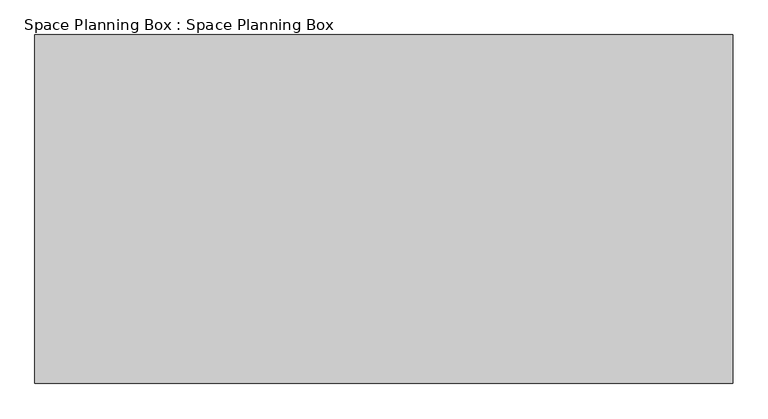
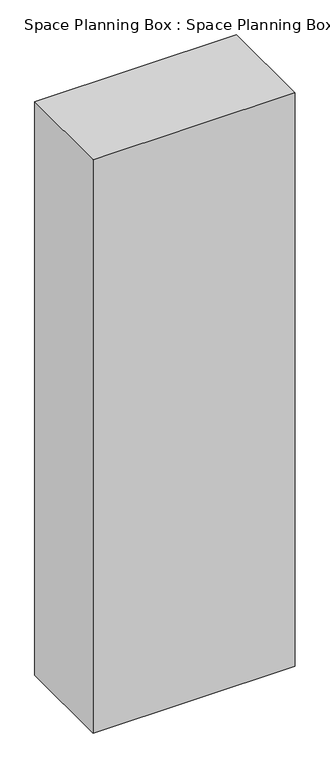
"""IFC4 building model written with IfcOpenShell, lengths in millimetres: proxy geometry, Space Planning Box : Space Planning Box."""

from ifc_helpers import new_model, si_unit, origin, origin_with_axes, place, context, project, spatial, polyline, outline, extrude, source, transform, mapped, element, save


def space_planning_box_space_planning_box_da00a96f(model_context):
    return source(origin(), model_context, "Body", "SweptSolid", [
        extrude(outline(polyline([(1000.0, 500.0), (1000.0, -500.0), (-1000.0, -500.0), (-1000.0, 500.0), (1000.0, 500.0)])), origin_with_axes(), (0.0, 0.0, 1.0), 6000.0),
    ])


if __name__ == "__main__":
    model = new_model("IFC4")
    model_context = context("Model", 3, world=origin())
    ifc_project = project(units=[si_unit("LENGTHUNIT", "METRE", prefix="MILLI")], contexts=[model_context])
    site = spatial("IfcSite", under=ifc_project)
    building = spatial("IfcBuilding", under=site)
    placement = place(None, origin())
    space_planning_box_space_planning_box_shape = space_planning_box_space_planning_box_da00a96f(model_context)
    element("IfcBuildingElementProxy", 1, Name="Space Planning Box : Space Planning Box", ObjectType="Space Planning Box : Space Planning Box", at=placement, inside=building, context=model_context, shape_type="MappedRepresentation", body=[
        mapped(space_planning_box_space_planning_box_shape, transform((0.0, 0.0, 0.0), x_axis=(1.0, 0.0, 0.0), y_axis=(0.0, 1.0, 0.0), z_axis=(0.0, 0.0, 1.0))),
    ])
    save(model, "model.ifc")

# Revit data of these elements
# Type "Space Planning Box : Space Planning Box"
#   Type Comments = "..."
#   Room Name [instance default] = "?"
#   Assembly Code = "..."
#   Width [instance default] = 1524 mm
#   Program Area [instance default] = 0 m²
#   Length [instance default] = 1524 mm
#   Height [instance default] = 1524 mm
#   Area [instance default] = 2.32258 m²
#   Fill Color [instance default] = Cyan
#   Default Elevation = 0
# Element 1 (IfcBuildingElementProxy, "Space Planning Box : Space Planning Box")
#   Room Name = "Corridor"
#   Width = 2000 mm
#   Length = 1000 mm
#   Height = 6000 mm
#   Area = 2 m²
#   Fill Color = Lavender
#   Materials on its faces: "Lavender"
# Materials
#   "Cyan": class "Generic", colour RGB 0 255 255, transparency 0.2, Cost = 0
#   "Lavender": class "Generic", colour RGB 186 85 211, transparency 0.2, Cost = 0
